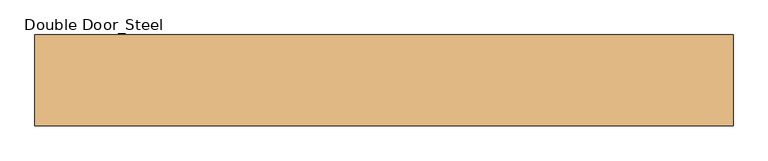
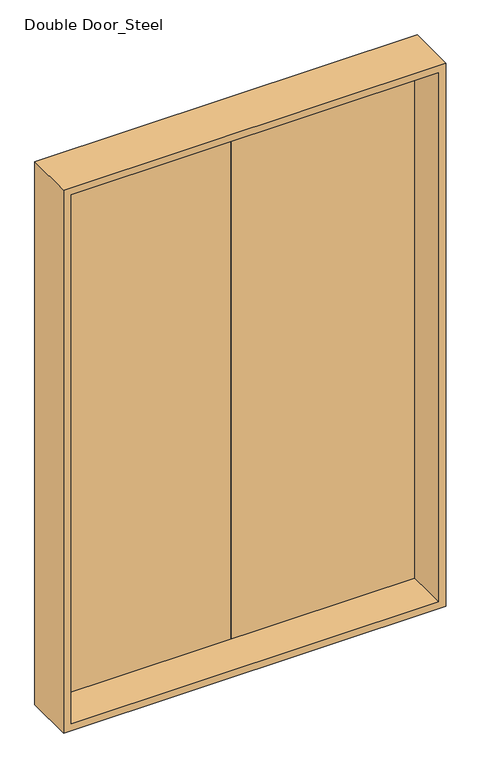
"""IFC4 building model written with IfcOpenShell, lengths in millimetres: door geometry, Double Door_Steel : H_DR_AMB_Double Door_Steel_W1800xH2700."""

from ifc_helpers import new_model, si_unit, frame, origin, place, context, project, spatial, polyline, outline, extrude, faceted_brep, source, transform, mapped, element, save


def double_door_steel_474d71af(model_context):
    return source(origin(), model_context, "Body", "SolidModel", [
        extrude(outline(polyline([(880.0, 77.0), (0.0, 77.0), (0.0, 117.0), (880.0, 117.0), (880.0, 77.0)])), frame((0.0, 0.0, 20.0), z_axis=(0.0, 0.0, 1.0), x_axis=(1.0, 0.0, 0.0)), (0.0, 0.0, 1.0), 2660.0),
        extrude(outline(polyline([(0.0, 77.0), (-880.0, 77.0), (-880.0, 117.0), (0.0, 117.0), (0.0, 77.0)])), frame((0.0, 0.0, 20.0), z_axis=(0.0, 0.0, 1.0), x_axis=(1.0, 0.0, 0.0)), (0.0, 0.0, 1.0), 2660.0),
        faceted_brep([(900.0, -117.0, 2700.0), (900.0, 117.0, 2700.0), (-900.0, 117.0, 2700.0), (-900.0, -117.0, 2700.0), (865.0, 77.0, 2665.0), (865.0, -117.0, 2665.0), (-865.0, -117.0, 2665.0), (-865.0, 77.0, 2665.0), (880.0, 117.0, 2680.0), (880.0, 77.0, 2680.0), (-880.0, 77.0, 2680.0), (-880.0, 117.0, 2680.0), (-900.0, 117.0, 0.0), (-900.0, -117.0, 0.0), (-865.0, -117.0, 35.0), (-865.0, 77.0, 35.0), (-880.0, 77.0, 20.0), (-880.0, 117.0, 20.0), (900.0, 117.0, 0.0), (880.0, 117.0, 20.0), (900.0, -117.0, 0.0), (865.0, -117.0, 35.0), (865.0, 77.0, 35.0), (880.0, 77.0, 20.0)], [[[0, 1, 2, 3]], [[4, 5, 6, 7]], [[8, 9, 10, 11]], [[3, 2, 12, 13]], [[7, 6, 14, 15]], [[11, 10, 16, 17]], [[18, 12, 2, 1], [8, 11, 17, 19]], [[13, 12, 18, 20]], [[0, 3, 13, 20], [21, 14, 6, 5]], [[15, 14, 21, 22]], [[23, 16, 10, 9], [4, 7, 15, 22]], [[17, 16, 23, 19]], [[20, 18, 1, 0]], [[22, 21, 5, 4]], [[19, 23, 9, 8]]]),
    ])


if __name__ == "__main__":
    model = new_model("IFC4")
    model_context = context("Model", 3, world=origin())
    ifc_project = project(units=[si_unit("LENGTHUNIT", "METRE", prefix="MILLI")], contexts=[model_context])
    site = spatial("IfcSite", under=ifc_project)
    building = spatial("IfcBuilding", under=site)
    placement = place(None, origin())
    double_door_steel_shape = double_door_steel_474d71af(model_context)
    element("IfcDoor", 1, ObjectType="Double Door_Steel : H_DR_AMB_Double Door_Steel_W1800xH2700", at=placement, inside=building, context=model_context, shape_type="MappedRepresentation", body=[
        mapped(double_door_steel_shape, transform((0.0, 0.0, 0.0), x_axis=(1.0, 0.0, 0.0), y_axis=(0.0, 1.0, 0.0), z_axis=(0.0, 0.0, 1.0))),
    ])
    save(model, "model.ifc")

# Revit data of these elements
# Type "Double Door_Steel : H_DR_AMB_Double Door_Steel_W1800xH2700"
#   Type Mark = "363"
#   프레임 = ""
#   철물 = ""
#   유리/마감 = ""
#   위치/개소 = ""
#   부호 = "1/SD"
#   문번호 = ""
#   문기호 = "SD"
#   Analytic Construction = "<None>"
#   Height = 2700.000 mm
#   Width = 1800.000 mm
#   Define Thermal Properties by = 1
#   문 틀 = none
#   문 = none
#   Function = (empty or 0)
#   Assembly Code = ""
#   Wall Closure = (empty or 0)
